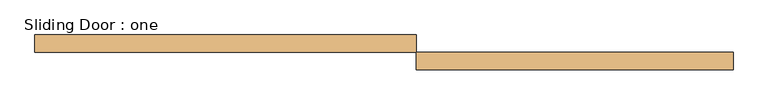
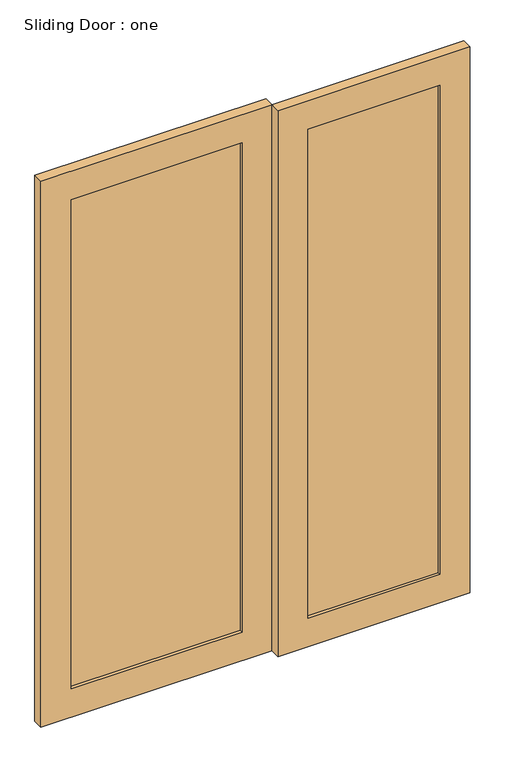
"""IFC4 building model written with IfcOpenShell, lengths in millimetres: door geometry, Sliding Door : one."""

import ifcopenshell
import ifcopenshell.guid

model = None  # the IFC model being written
_history = None  # IfcOwnerHistory: only IFC2X3 demands one
_inside = {}  # id of a spatial element -> (the spatial element, [elements in it])
_under = {}  # id of a project, library or spatial element -> (it, [spatial elements below it])
_declared = {}  # id of a project -> (the project, [libraries it declares])
_typed = {}  # id of a type object -> (the type object, [elements of that type])
_made_of = {}  # id of a material, layer set ... -> (it, [elements and type objects made of it])


def new_model(schema):
    """Start an empty IFC model of exactly this schema.

    Asked for "IFC4X3", IfcOpenShell would pick the latest addendum, in which some entities
    have other attributes; the version numbers below select the first issue.
    IFC2X3 requires an IfcOwnerHistory on every rooted entity: one is made here for all.
    """
    global model, _history
    if schema == "IFC4X3":
        model = ifcopenshell.file(schema_version=(4, 3, 0, 0))
    else:
        model = ifcopenshell.file(schema=schema)
    _inside.clear()
    _under.clear()
    _declared.clear()
    _typed.clear()
    _made_of.clear()
    _history = None
    if model.schema == "IFC2X3":
        org = make("IfcOrganization", Name="unknown")
        user = make(
            "IfcPersonAndOrganization",
            ThePerson=make("IfcPerson", FamilyName="unknown"),
            TheOrganization=org,
        )
        app = make(
            "IfcApplication",
            ApplicationDeveloper=org,
            Version="unknown",
            ApplicationFullName="unknown",
            ApplicationIdentifier="unknown",
        )
        _history = make(
            "IfcOwnerHistory",
            OwningUser=user,
            OwningApplication=app,
            ChangeAction="ADDED",
            CreationDate=0,
        )
    return model


def make(cls, **values):
    """One entity of the class cls with the attributes given. An attribute that is None is left unset."""
    return model.create_entity(
        cls, **{name: value for name, value in values.items() if value is not None}
    )


def rooted(cls, **values):
    """An entity with a GlobalId (a new one), such as an element, a storey or a relation."""
    return make(cls, GlobalId=ifcopenshell.guid.new(), OwnerHistory=_history, **values)


def si_unit(unit_type, name, prefix=None):
    """IfcSIUnit, for example si_unit("LENGTHUNIT", "METRE", prefix="MILLI")."""
    return make("IfcSIUnit", UnitType=unit_type, Prefix=prefix, Name=name)


def assignment(units):
    """IfcUnitAssignment: the units of a project."""
    return None if units is None else make("IfcUnitAssignment", Units=units)


def point(xyz):
    """IfcCartesianPoint."""
    return None if xyz is None else make("IfcCartesianPoint", Coordinates=xyz)


def direction(xyz):
    """IfcDirection."""
    return None if xyz is None else make("IfcDirection", DirectionRatios=xyz)


def frame(location, z_axis=None, x_axis=None):
    """IfcAxis2Placement3D, a coordinate frame: its origin and axes. An axis left out is left unset."""
    return make(
        "IfcAxis2Placement3D",
        Location=point(location),
        Axis=direction(z_axis),
        RefDirection=direction(x_axis),
    )


def origin():
    """The frame at (0, 0, 0) with its axes left unset."""
    return frame((0.0, 0.0, 0.0))


def place(relative_to, where):
    """IfcLocalPlacement: puts the frame where relative to a parent placement (None: the world)."""
    return make(
        "IfcLocalPlacement", PlacementRelTo=relative_to, RelativePlacement=where
    )


def context(
    kind, dimensions, precision=None, world=None, true_north=None, identifier=None
):
    """IfcGeometricRepresentationContext, for example the 3D "Model" context."""
    return make(
        "IfcGeometricRepresentationContext",
        ContextIdentifier=identifier,
        ContextType=kind,
        CoordinateSpaceDimension=dimensions,
        Precision=precision,
        WorldCoordinateSystem=world,
        TrueNorth=true_north,
    )


def project(units=None, contexts=None):
    """IfcProject with its units and contexts."""
    return rooted(
        "IfcProject",
        Name="project",
        RepresentationContexts=contexts,
        UnitsInContext=assignment(units),
    )


def spatial(cls, under=None, at=None, **own):
    """A site, building, storey or space (cls), placed at a placement, below another one or the project."""
    s = rooted(cls, ObjectPlacement=at, **own)
    if under is not None:
        _under.setdefault(under.id(), (under, []))[1].append(s)
    return s


def polyline(points):
    """IfcPolyline through the points."""
    return make("IfcPolyline", Points=[point(p) for p in points])


def outline(outer, holes=None, kind="AREA"):
    """IfcArbitraryClosedProfileDef: a profile drawn as a closed curve; with holes, ...WithVoids."""
    if holes is None:
        return make("IfcArbitraryClosedProfileDef", ProfileType=kind, OuterCurve=outer)
    return make(
        "IfcArbitraryProfileDefWithVoids",
        ProfileType=kind,
        OuterCurve=outer,
        InnerCurves=holes,
    )


def extrude(swept, where, along, depth):
    """IfcExtrudedAreaSolid: the profile swept, set in the frame where, extruded along a direction by depth."""
    return make(
        "IfcExtrudedAreaSolid",
        SweptArea=swept,
        Position=where,
        ExtrudedDirection=direction(along),
        Depth=depth,
    )


def shape(context_of_items, identifier, shape_type, items):
    """IfcShapeRepresentation: the items that make up one representation, for example the "Body"."""
    return make(
        "IfcShapeRepresentation",
        ContextOfItems=context_of_items,
        RepresentationIdentifier=identifier,
        RepresentationType=shape_type,
        Items=items,
    )


def source(mapping_origin, context_of_items, identifier, shape_type, items):
    """IfcRepresentationMap: a shape defined once, which mapped items show again and again."""
    return make(
        "IfcRepresentationMap",
        MappingOrigin=mapping_origin,
        MappedRepresentation=shape(context_of_items, identifier, shape_type, items),
    )


def transform(
    local_origin,
    x_axis=None,
    y_axis=None,
    z_axis=None,
    scale=None,
    scale2=None,
    scale3=None,
    uniform=True,
):
    """IfcCartesianTransformationOperator3D, or its non-uniform kind. x_axis, y_axis, z_axis: its Axis1, 2, 3."""
    if uniform:
        return make(
            "IfcCartesianTransformationOperator3D",
            Axis1=direction(x_axis),
            Axis2=direction(y_axis),
            LocalOrigin=point(local_origin),
            Scale=scale,
            Axis3=direction(z_axis),
        )
    return make(
        "IfcCartesianTransformationOperator3DnonUniform",
        Axis1=direction(x_axis),
        Axis2=direction(y_axis),
        LocalOrigin=point(local_origin),
        Scale=scale,
        Axis3=direction(z_axis),
        Scale2=scale2,
        Scale3=scale3,
    )


def mapped(mapping_source, mapping_target):
    """IfcMappedItem: shows the shape of a source again, moved by a transform."""
    return make(
        "IfcMappedItem", MappingSource=mapping_source, MappingTarget=mapping_target
    )


def made_of(thing, what):
    """Note that an element or type object is made of a material, layer set ...; save() writes the relation."""
    if what is not None:
        _made_of.setdefault(what.id(), (what, []))[1].append(thing)
    return thing


def element(
    cls,
    number,
    at=None,
    inside=None,
    cuts=None,
    type_object=None,
    material=None,
    context=None,
    identifier="Body",
    shape_type=None,
    held_by="IfcProductDefinitionShape",
    body=None,
    shapes=None,
    **own,
):
    """One element of the class cls, such as IfcWall. Its Tag is "e" and its number.

    at: its placement. inside: the storey or other place that contains it. cuts: it is an
    opening in that element (IfcRelVoidsElement). A single representation is given by context,
    identifier, shape_type and body (its items); several are given by shapes. held_by: the class
    of the entity that holds the representations. save() writes the other relations.
    """
    e = rooted(cls, Tag="e%d" % number, ObjectPlacement=at, **own)
    if body is not None:
        shapes = [shape(context, identifier, shape_type, body)]
    if shapes is not None:
        e.Representation = make(held_by, Representations=shapes)
    if inside is not None:
        _inside.setdefault(inside.id(), (inside, []))[1].append(e)
    if cuts is not None:
        rooted(
            "IfcRelVoidsElement", RelatingBuildingElement=cuts, RelatedOpeningElement=e
        )
    if type_object is not None:
        _typed.setdefault(type_object.id(), (type_object, []))[1].append(e)
    return made_of(e, material)


def aggregate(whole, parts):
    """IfcRelAggregates: a whole, such as a stair, and the parts it consists of."""
    return rooted("IfcRelAggregates", RelatingObject=whole, RelatedObjects=parts)


def save(model, path):
    """Write the relations noted so far, then the file.

    IfcRelAggregates (storeys below a building ...), IfcRelContainedInSpatialStructure (elements
    in a storey), IfcRelDefinesByType, IfcRelAssociatesMaterial and IfcRelDeclares: one each for
    every whole, place, type object, material and project.
    """
    for whole, parts in _under.values():
        aggregate(whole, parts)
    for where, things in _inside.values():
        rooted(
            "IfcRelContainedInSpatialStructure",
            RelatedElements=things,
            RelatingStructure=where,
        )
    for kind, things in _typed.values():
        rooted("IfcRelDefinesByType", RelatedObjects=things, RelatingType=kind)
    for what, things in _made_of.values():
        rooted("IfcRelAssociatesMaterial", RelatedObjects=things, RelatingMaterial=what)
    for by, libraries in _declared.values():
        rooted("IfcRelDeclares", RelatingContext=by, RelatedDefinitions=libraries)
    model.write(path)


def sliding_door_one_977cb0c7(model_context):
    return source(origin(), model_context, "Body", "SweptSolid", [
        extrude(outline(polyline([(-44.4768999, 50.8), (-44.4768999, 31.75), (-766.7625, 31.75), (-766.7625, 50.8), (-44.4768999, 50.8)])), frame((0.0, 0.0, 127.0), z_axis=(0.0, 0.0, 1.0), x_axis=(1.0, 0.0, 0.0)), (0.0, 0.0, 1.0), 2184.4),
        extrude(outline(polyline([(766.7625, 6.35), (766.7625, -12.7), (209.5231001, -12.7), (209.5231001, 6.35), (766.7625, 6.35)])), frame((0.0, 0.0, 127.0), z_axis=(0.0, 0.0, 1.0), x_axis=(1.0, 0.0, 0.0)), (0.0, 0.0, 1.0), 2184.4),
        extrude(outline(polyline([(2438.4, -893.7625), (0.0, -893.7625), (0.0, 82.5231001), (2438.4, 82.5231001), (2438.4, -893.7625)]), holes=[polyline([(127.0, -44.4768999), (127.0, -766.7625), (2311.4, -766.7625), (2311.4, -44.4768999), (127.0, -44.4768999)])]), frame((0.0, 19.05, 0.0), z_axis=(0.0, 1.0, 0.0), x_axis=(0.0, 0.0, 1.0)), (0.0, 0.0, 1.0), 44.45),
        extrude(outline(polyline([(2438.4, 82.5231001), (0.0, 82.5231001), (0.0, 893.7625), (2438.4, 893.7625), (2438.4, 82.5231001)]), holes=[polyline([(127.0, 766.7625), (127.0, 209.5231001), (2311.4, 209.5231001), (2311.4, 766.7625), (127.0, 766.7625)])]), frame((0.0, -25.4, 0.0), z_axis=(0.0, 1.0, 0.0), x_axis=(0.0, 0.0, 1.0)), (0.0, 0.0, 1.0), 44.45),
    ])


if __name__ == "__main__":
    model = new_model("IFC4")
    model_context = context("Model", 3, world=origin())
    ifc_project = project(units=[si_unit("LENGTHUNIT", "METRE", prefix="MILLI")], contexts=[model_context])
    site = spatial("IfcSite", under=ifc_project)
    building = spatial("IfcBuilding", under=site)
    placement = place(None, origin())
    sliding_door_one_shape = sliding_door_one_977cb0c7(model_context)
    element("IfcDoor", 1, ObjectType="Sliding Door : one", at=placement, inside=building, context=model_context, shape_type="MappedRepresentation", body=[
        mapped(sliding_door_one_shape, transform((0.0, 0.0, 0.0), x_axis=(1.0, 0.0, 0.0), y_axis=(0.0, 1.0, 0.0), z_axis=(0.0, 0.0, 1.0))),
    ])
    save(model, "model.ifc")

# Revit data of these elements
# Type "Sliding Door : one"
#   Type Mark = "42"
#   Analytic Construction = "<None>"
#   Stile_Width = 0' - 5"
#   Door_Thickness = 0' - 1 3/4"
#   Door_Offset = 0' - 1"
#   Glass_Material = SAFETY GLAZING
#   Frame_Material = INTERIOR GRADE ALUMINUM STOREFRONT W/ SAFETY GLAZING
#   Function = (empty or 0)
# Element 1 (IfcDoor, "Sliding Door : one")
#   Materials on its faces: "INTERIOR GRADE ALUMINUM STOREFRONT W/ SAFETY GLAZING", "SAFETY GLAZING"
# Materials
#   "SAFETY GLAZING": class "Glass", colour RGB 142 168 196, transparency 0.75, Description = "Soda Lime Glass", Cost = 0
#   "INTERIOR GRADE ALUMINUM STOREFRONT W/ SAFETY GLAZING": class "Metal", colour RGB 226 226 226, transparency 0, Description = "Aluminum 6061", Cost = 0
